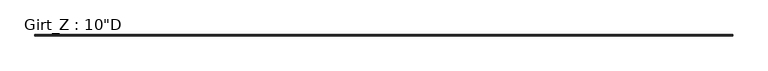
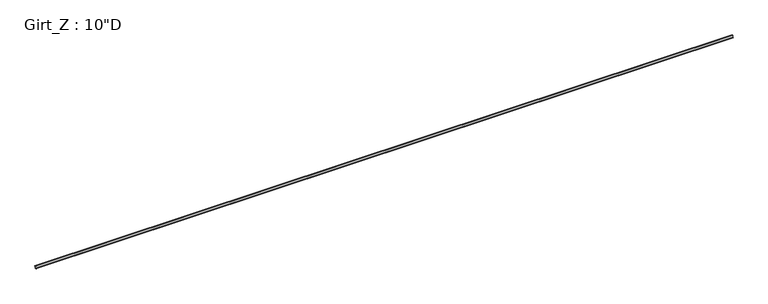
"""IFC4 building model written with IfcOpenShell, lengths in millimetres: beam geometry."""

from ifc_helpers import new_model, si_unit, point, frame, frame_2d, origin, place, context, project, spatial, polyline, circle_curve, trimmed, segment, composite_curve, outline, extrude, source, transform, mapped, element, save


def beam_628135af(model_context):
    return source(origin(), model_context, "Body", "SweptSolid", [
        extrude(outline(composite_curve([segment(polyline([(63.5, 127.0), (75.745104, 112.4068534), (73.6169367, 110.621109), (62.204539, 124.221875), (3.3005807, 124.221875)]), True, "CONTINUOUS"), segment(trimmed(circle_curve(frame_2d((3.3741066, 122.2381931)), 1.9850441), [point((3.3005807, 124.221875))], [point((1.3890625, 122.2381931))], True, "CARTESIAN"), True, "CONTINUOUS"), segment(polyline([(1.3890625, 122.2381931), (1.3890625, -122.2375)]), True, "CONTINUOUS"), segment(trimmed(circle_curve(frame_2d((-3.3734375, -122.2375)), 4.7625), [point((1.3890625, -122.2375))], [point((-3.3734375, -127.0))], False, "CARTESIAN"), True, "CONTINUOUS"), segment(polyline([(-3.3734375, -127.0), (-63.5, -127.0), (-75.745104, -112.4068534), (-73.6169367, -110.621109), (-62.204539, -124.221875), (-3.2694106, -124.221875)]), True, "CONTINUOUS"), segment(trimmed(circle_curve(frame_2d((-3.3748024, -122.2389339)), 1.9857399), [point((-3.2694106, -124.221875))], [point((-1.3890625, -122.2389339))], True, "CARTESIAN"), True, "CONTINUOUS"), segment(polyline([(-1.3890625, -122.2389339), (-1.3890625, 122.2375)]), True, "CONTINUOUS"), segment(trimmed(circle_curve(frame_2d((3.3734375, 122.2375)), 4.7625), [point((-1.3890625, 122.2375))], [point((3.3734375, 127.0))], False, "CARTESIAN"), True, "CONTINUOUS"), segment(polyline([(3.3734375, 127.0), (63.5, 127.0)]), True, "CONTINUOUS")], self_intersect=False)), frame((-40443.15, 0.0, 0.0), z_axis=(1.0, 0.0, 0.0), x_axis=(0.0, 1.0, 0.0)), (0.0, 0.0, 1.0), 80644.9999998),
    ])


if __name__ == "__main__":
    model = new_model("IFC4")
    model_context = context("Model", 3, world=origin())
    ifc_project = project(units=[si_unit("LENGTHUNIT", "METRE", prefix="MILLI")], contexts=[model_context])
    site = spatial("IfcSite", under=ifc_project)
    building = spatial("IfcBuilding", under=site)
    placement = place(None, origin())
    beam_shape = beam_628135af(model_context)
    element("IfcBeam", 1, ObjectType="Girt_Z : 10\"D", at=placement, inside=building, context=model_context, shape_type="MappedRepresentation", body=[
        mapped(beam_shape, transform((0.0, 0.0, 0.0), x_axis=(1.0, 0.0, 0.0), y_axis=(0.0, 1.0, 0.0), z_axis=(0.0, 0.0, 1.0))),
    ])
    save(model, "model.ifc")

# Revit data of these elements
# Type "Girt_Z : 10\"D"
#   Web_Thickness = 0' - 0 7/64"
#   Length [instance default] = 10' - 0"
#   Leg_1 = 0' - 2 1/2"
#   Height = 0' - 10"
#   Structural Material [instance default] = none
